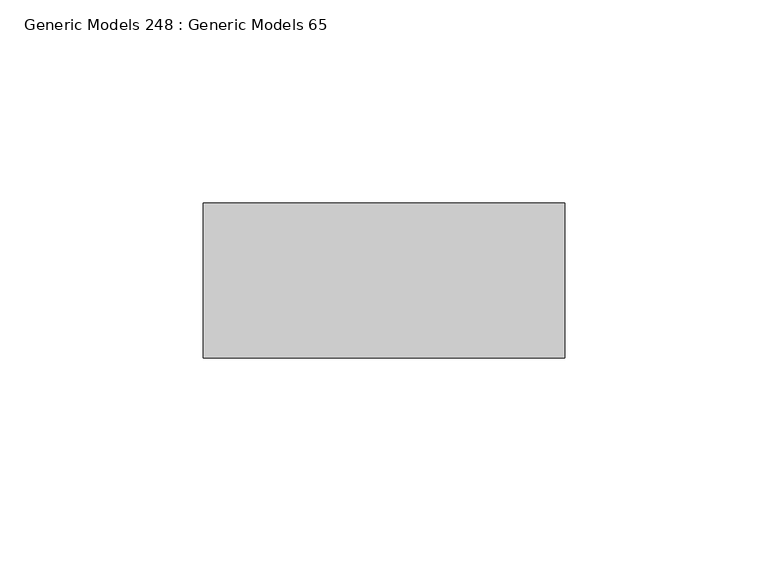
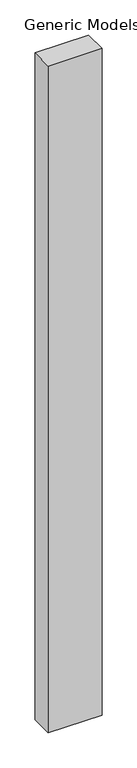
"""IFC4 building model written with IfcOpenShell, lengths in millimetres: proxy geometry, Generic Models 248 : Generic Models 65."""

import ifcopenshell
import ifcopenshell.guid

model = None  # the IFC model being written
_history = None  # IfcOwnerHistory: only IFC2X3 demands one
_inside = {}  # id of a spatial element -> (the spatial element, [elements in it])
_under = {}  # id of a project, library or spatial element -> (it, [spatial elements below it])
_declared = {}  # id of a project -> (the project, [libraries it declares])
_typed = {}  # id of a type object -> (the type object, [elements of that type])
_made_of = {}  # id of a material, layer set ... -> (it, [elements and type objects made of it])


def new_model(schema):
    """Start an empty IFC model of exactly this schema.

    Asked for "IFC4X3", IfcOpenShell would pick the latest addendum, in which some entities
    have other attributes; the version numbers below select the first issue.
    IFC2X3 requires an IfcOwnerHistory on every rooted entity: one is made here for all.
    """
    global model, _history
    if schema == "IFC4X3":
        model = ifcopenshell.file(schema_version=(4, 3, 0, 0))
    else:
        model = ifcopenshell.file(schema=schema)
    _inside.clear()
    _under.clear()
    _declared.clear()
    _typed.clear()
    _made_of.clear()
    _history = None
    if model.schema == "IFC2X3":
        org = make("IfcOrganization", Name="unknown")
        user = make(
            "IfcPersonAndOrganization",
            ThePerson=make("IfcPerson", FamilyName="unknown"),
            TheOrganization=org,
        )
        app = make(
            "IfcApplication",
            ApplicationDeveloper=org,
            Version="unknown",
            ApplicationFullName="unknown",
            ApplicationIdentifier="unknown",
        )
        _history = make(
            "IfcOwnerHistory",
            OwningUser=user,
            OwningApplication=app,
            ChangeAction="ADDED",
            CreationDate=0,
        )
    return model


def make(cls, **values):
    """One entity of the class cls with the attributes given. An attribute that is None is left unset."""
    return model.create_entity(
        cls, **{name: value for name, value in values.items() if value is not None}
    )


def rooted(cls, **values):
    """An entity with a GlobalId (a new one), such as an element, a storey or a relation."""
    return make(cls, GlobalId=ifcopenshell.guid.new(), OwnerHistory=_history, **values)


def si_unit(unit_type, name, prefix=None):
    """IfcSIUnit, for example si_unit("LENGTHUNIT", "METRE", prefix="MILLI")."""
    return make("IfcSIUnit", UnitType=unit_type, Prefix=prefix, Name=name)


def assignment(units):
    """IfcUnitAssignment: the units of a project."""
    return None if units is None else make("IfcUnitAssignment", Units=units)


def point(xyz):
    """IfcCartesianPoint."""
    return None if xyz is None else make("IfcCartesianPoint", Coordinates=xyz)


def direction(xyz):
    """IfcDirection."""
    return None if xyz is None else make("IfcDirection", DirectionRatios=xyz)


def frame(location, z_axis=None, x_axis=None):
    """IfcAxis2Placement3D, a coordinate frame: its origin and axes. An axis left out is left unset."""
    return make(
        "IfcAxis2Placement3D",
        Location=point(location),
        Axis=direction(z_axis),
        RefDirection=direction(x_axis),
    )


def origin():
    """The frame at (0, 0, 0) with its axes left unset."""
    return frame((0.0, 0.0, 0.0))


def place(relative_to, where):
    """IfcLocalPlacement: puts the frame where relative to a parent placement (None: the world)."""
    return make(
        "IfcLocalPlacement", PlacementRelTo=relative_to, RelativePlacement=where
    )


def context(
    kind, dimensions, precision=None, world=None, true_north=None, identifier=None
):
    """IfcGeometricRepresentationContext, for example the 3D "Model" context."""
    return make(
        "IfcGeometricRepresentationContext",
        ContextIdentifier=identifier,
        ContextType=kind,
        CoordinateSpaceDimension=dimensions,
        Precision=precision,
        WorldCoordinateSystem=world,
        TrueNorth=true_north,
    )


def project(units=None, contexts=None):
    """IfcProject with its units and contexts."""
    return rooted(
        "IfcProject",
        Name="project",
        RepresentationContexts=contexts,
        UnitsInContext=assignment(units),
    )


def spatial(cls, under=None, at=None, **own):
    """A site, building, storey or space (cls), placed at a placement, below another one or the project."""
    s = rooted(cls, ObjectPlacement=at, **own)
    if under is not None:
        _under.setdefault(under.id(), (under, []))[1].append(s)
    return s


def polyline(points):
    """IfcPolyline through the points."""
    return make("IfcPolyline", Points=[point(p) for p in points])


def outline(outer, holes=None, kind="AREA"):
    """IfcArbitraryClosedProfileDef: a profile drawn as a closed curve; with holes, ...WithVoids."""
    if holes is None:
        return make("IfcArbitraryClosedProfileDef", ProfileType=kind, OuterCurve=outer)
    return make(
        "IfcArbitraryProfileDefWithVoids",
        ProfileType=kind,
        OuterCurve=outer,
        InnerCurves=holes,
    )


def extrude(swept, where, along, depth):
    """IfcExtrudedAreaSolid: the profile swept, set in the frame where, extruded along a direction by depth."""
    return make(
        "IfcExtrudedAreaSolid",
        SweptArea=swept,
        Position=where,
        ExtrudedDirection=direction(along),
        Depth=depth,
    )


def shape(context_of_items, identifier, shape_type, items):
    """IfcShapeRepresentation: the items that make up one representation, for example the "Body"."""
    return make(
        "IfcShapeRepresentation",
        ContextOfItems=context_of_items,
        RepresentationIdentifier=identifier,
        RepresentationType=shape_type,
        Items=items,
    )


def source(mapping_origin, context_of_items, identifier, shape_type, items):
    """IfcRepresentationMap: a shape defined once, which mapped items show again and again."""
    return make(
        "IfcRepresentationMap",
        MappingOrigin=mapping_origin,
        MappedRepresentation=shape(context_of_items, identifier, shape_type, items),
    )


def transform(
    local_origin,
    x_axis=None,
    y_axis=None,
    z_axis=None,
    scale=None,
    scale2=None,
    scale3=None,
    uniform=True,
):
    """IfcCartesianTransformationOperator3D, or its non-uniform kind. x_axis, y_axis, z_axis: its Axis1, 2, 3."""
    if uniform:
        return make(
            "IfcCartesianTransformationOperator3D",
            Axis1=direction(x_axis),
            Axis2=direction(y_axis),
            LocalOrigin=point(local_origin),
            Scale=scale,
            Axis3=direction(z_axis),
        )
    return make(
        "IfcCartesianTransformationOperator3DnonUniform",
        Axis1=direction(x_axis),
        Axis2=direction(y_axis),
        LocalOrigin=point(local_origin),
        Scale=scale,
        Axis3=direction(z_axis),
        Scale2=scale2,
        Scale3=scale3,
    )


def mapped(mapping_source, mapping_target):
    """IfcMappedItem: shows the shape of a source again, moved by a transform."""
    return make(
        "IfcMappedItem", MappingSource=mapping_source, MappingTarget=mapping_target
    )


def made_of(thing, what):
    """Note that an element or type object is made of a material, layer set ...; save() writes the relation."""
    if what is not None:
        _made_of.setdefault(what.id(), (what, []))[1].append(thing)
    return thing


def element(
    cls,
    number,
    at=None,
    inside=None,
    cuts=None,
    type_object=None,
    material=None,
    context=None,
    identifier="Body",
    shape_type=None,
    held_by="IfcProductDefinitionShape",
    body=None,
    shapes=None,
    **own,
):
    """One element of the class cls, such as IfcWall. Its Tag is "e" and its number.

    at: its placement. inside: the storey or other place that contains it. cuts: it is an
    opening in that element (IfcRelVoidsElement). A single representation is given by context,
    identifier, shape_type and body (its items); several are given by shapes. held_by: the class
    of the entity that holds the representations. save() writes the other relations.
    """
    e = rooted(cls, Tag="e%d" % number, ObjectPlacement=at, **own)
    if body is not None:
        shapes = [shape(context, identifier, shape_type, body)]
    if shapes is not None:
        e.Representation = make(held_by, Representations=shapes)
    if inside is not None:
        _inside.setdefault(inside.id(), (inside, []))[1].append(e)
    if cuts is not None:
        rooted(
            "IfcRelVoidsElement", RelatingBuildingElement=cuts, RelatedOpeningElement=e
        )
    if type_object is not None:
        _typed.setdefault(type_object.id(), (type_object, []))[1].append(e)
    return made_of(e, material)


def aggregate(whole, parts):
    """IfcRelAggregates: a whole, such as a stair, and the parts it consists of."""
    return rooted("IfcRelAggregates", RelatingObject=whole, RelatedObjects=parts)


def save(model, path):
    """Write the relations noted so far, then the file.

    IfcRelAggregates (storeys below a building ...), IfcRelContainedInSpatialStructure (elements
    in a storey), IfcRelDefinesByType, IfcRelAssociatesMaterial and IfcRelDeclares: one each for
    every whole, place, type object, material and project.
    """
    for whole, parts in _under.values():
        aggregate(whole, parts)
    for where, things in _inside.values():
        rooted(
            "IfcRelContainedInSpatialStructure",
            RelatedElements=things,
            RelatingStructure=where,
        )
    for kind, things in _typed.values():
        rooted("IfcRelDefinesByType", RelatedObjects=things, RelatingType=kind)
    for what, things in _made_of.values():
        rooted("IfcRelAssociatesMaterial", RelatedObjects=things, RelatingMaterial=what)
    for by, libraries in _declared.values():
        rooted("IfcRelDeclares", RelatingContext=by, RelatedDefinitions=libraries)
    model.write(path)


def generic_models_248_generic_models_65_f6c484d7(model_context):
    return source(origin(), model_context, "Body", "SweptSolid", [
        extrude(outline(polyline([(47345.6, 592.1375), (47256.7, 592.1375), (47256.7, 630.2375), (47345.6, 630.2375), (47345.6, 592.1375)])), frame((0.0, 0.0, 4305.3), z_axis=(0.0, 0.0, 1.0), x_axis=(1.0, 0.0, 0.0)), (0.0, 0.0, 1.0), 1162.05),
    ])


if __name__ == "__main__":
    model = new_model("IFC4")
    model_context = context("Model", 3, world=origin())
    ifc_project = project(units=[si_unit("LENGTHUNIT", "METRE", prefix="MILLI")], contexts=[model_context])
    site = spatial("IfcSite", under=ifc_project)
    building = spatial("IfcBuilding", under=site)
    placement = place(None, origin())
    generic_models_248_generic_models_65_shape = generic_models_248_generic_models_65_f6c484d7(model_context)
    element("IfcBuildingElementProxy", 1, Name="Generic Models 248 : Generic Models 65", ObjectType="Generic Models 248 : Generic Models 65", at=placement, inside=building, context=model_context, shape_type="MappedRepresentation", body=[
        mapped(generic_models_248_generic_models_65_shape, transform((0.0, 0.0, 0.0), x_axis=(1.0, 0.0, 0.0), y_axis=(0.0, 1.0, 0.0), z_axis=(0.0, 0.0, 1.0))),
    ])
    save(model, "model.ifc")

# Revit data of these elements
# Element 1 (IfcBuildingElementProxy, "Generic Models 248 : Generic Models 65")
#   Materials on its faces: "2X WOOD STUD - SEE 'WALL TAG' & 'LAYER MATERIAL SCHEDULE' FOR SPACING & INSULATION TREATMENT, IF APPLICAPLE"
# Materials
#   "2X WOOD STUD - SEE 'WALL TAG' & 'LAYER MATERIAL SCHEDULE' FOR SPACING & INSULATION TREATMENT, IF APPLICAPLE": class "Wood", colour RGB 234 198 147, transparency 0, Description = "Pinus Echinata", Cost = 0
